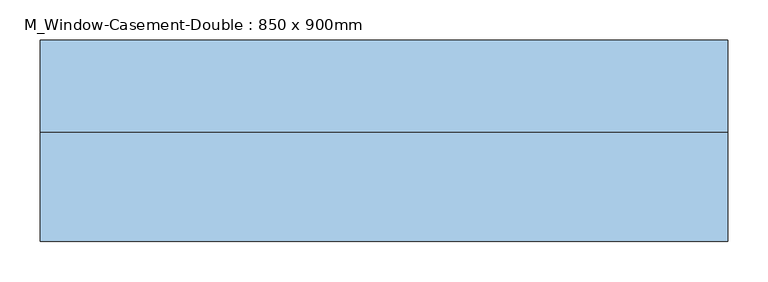
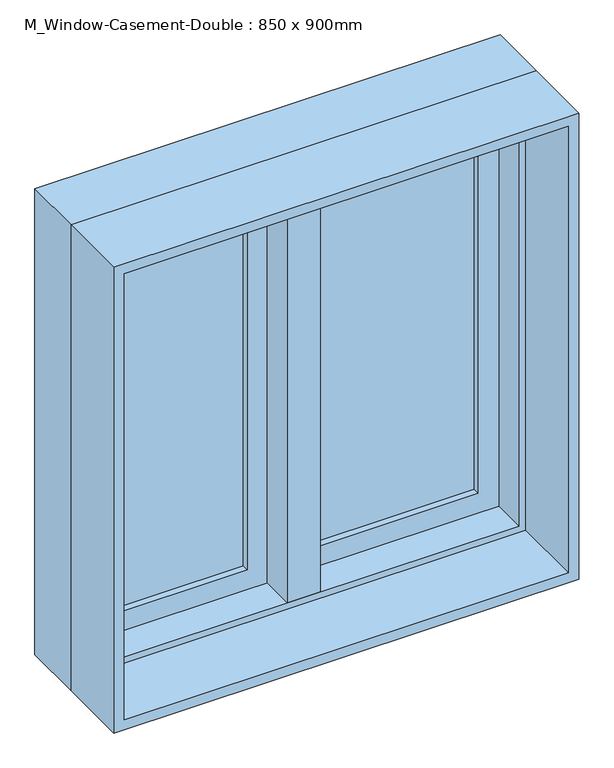
"""IFC4 building model written with IfcOpenShell, lengths in millimetres: window geometry, M_Window-Casement-Double : 850 x 900mm."""

from ifc_helpers import new_model, si_unit, frame, origin, place, context, project, spatial, polyline, outline, extrude, faceted_brep, source, transform, mapped, element, save


def m_window_casement_double_850_x_900mm_c1c4159e(model_context):
    return source(origin(), model_context, "Body", "SolidModel", [
        faceted_brep([(9.525, 134.05, 1787.3), (-9.525, 134.05, 1787.3), (-9.525, 83.25, 1787.3), (9.525, 83.25, 1787.3), (9.525, 134.05, 912.7), (9.525, 83.25, 912.7), (-9.525, 83.25, 912.7), (-9.525, 134.05, 912.7), (-9.525, 83.25, 931.75), (-9.525, 83.25, 1768.25), (-30.1625, 83.25, 931.75), (-30.1625, 83.25, 1768.25), (-30.1625, 19.75, 931.75), (-30.1625, 19.75, 1768.25), (30.1625, 19.75, 931.75), (30.1625, 19.75, 1768.25), (30.1625, 83.25, 931.75), (30.1625, 83.25, 1768.25), (9.525, 83.25, 931.75), (9.525, 83.25, 1768.25)], [[[0, 1, 2, 3]], [[4, 5, 6, 7]], [[1, 0, 4, 7]], [[2, 1, 7, 6, 8, 9]], [[9, 8, 10, 11]], [[11, 10, 12, 13]], [[13, 12, 14, 15]], [[15, 14, 16, 17]], [[17, 16, 18, 19]], [[0, 3, 19, 18, 5, 4]], [[18, 8, 6, 5]], [[9, 19, 3, 2]], [[8, 18, 16, 14, 12, 10]], [[19, 9, 11, 13, 15, 17]]]),
        extrude(outline(polyline([(-66.675, 115.0), (-66.675, 108.65), (-355.15, 108.65), (-355.15, 115.0), (-66.675, 115.0)])), frame((0.0, 0.0, 969.85), z_axis=(0.0, 0.0, 1.0), x_axis=(1.0, 0.0, 0.0)), (0.0, 0.0, 1.0), 760.3),
        extrude(outline(polyline([(-355.15, 95.95), (-355.15, 102.3), (-66.675, 102.3), (-66.675, 95.95), (-355.15, 95.95)])), frame((0.0, 0.0, 969.85), z_axis=(0.0, 0.0, 1.0), x_axis=(1.0, 0.0, 0.0)), (0.0, 0.0, 1.0), 760.3),
        extrude(outline(polyline([(355.15, 115.0), (355.15, 108.65), (66.675, 108.65), (66.675, 115.0), (355.15, 115.0)])), frame((0.0, 0.0, 969.85), z_axis=(0.0, 0.0, 1.0), x_axis=(1.0, 0.0, 0.0)), (0.0, 0.0, 1.0), 760.3),
        extrude(outline(polyline([(66.675, 95.95), (66.675, 102.3), (355.15, 102.3), (355.15, 95.95), (66.675, 95.95)])), frame((0.0, 0.0, 969.85), z_axis=(0.0, 0.0, 1.0), x_axis=(1.0, 0.0, 0.0)), (0.0, 0.0, 1.0), 760.3),
        extrude(outline(polyline([(1787.3, -412.3), (912.7, -412.3), (912.7, -9.525), (1787.3, -9.525), (1787.3, -412.3)]), holes=[polyline([(1730.15, -66.675), (969.85, -66.675), (969.85, -355.15), (1730.15, -355.15), (1730.15, -66.675)])]), frame((0.0, 83.25, 0.0), z_axis=(0.0, 1.0, 0.0), x_axis=(0.0, 0.0, 1.0)), (0.0, 0.0, 1.0), 44.45),
        extrude(outline(polyline([(912.7, 412.3), (1787.3, 412.3), (1787.3, 9.525), (912.7, 9.525), (912.7, 412.3)]), holes=[polyline([(969.85, 66.675), (1730.15, 66.675), (1730.15, 355.15), (969.85, 355.15), (969.85, 66.675)])]), frame((0.0, 83.25, 0.0), z_axis=(0.0, 1.0, 0.0), x_axis=(0.0, 0.0, 1.0)), (0.0, 0.0, 1.0), 44.45),
        extrude(outline(polyline([(1800.0, -425.0), (900.0, -425.0), (900.0, 425.0), (1800.0, 425.0), (1800.0, -425.0)]), holes=[polyline([(1780.95, 405.95), (919.05, 405.95), (919.05, -405.95), (1780.95, -405.95), (1780.95, 405.95)])]), frame((0.0, -115.0, 0.0), z_axis=(0.0, 1.0, 0.0), x_axis=(0.0, 0.0, 1.0)), (0.0, 0.0, 1.0), 134.75),
        faceted_brep([(393.25, 83.25, 1768.25), (393.25, 19.75, 1768.25), (-393.25, 19.75, 1768.25), (-393.25, 83.25, 1768.25), (412.3, 134.05, 1787.3), (412.3, 83.25, 1787.3), (-412.3, 83.25, 1787.3), (-412.3, 134.05, 1787.3), (425.0, 19.75, 1800.0), (425.0, 134.05, 1800.0), (-425.0, 134.05, 1800.0), (-425.0, 19.75, 1800.0), (-393.25, 19.75, 931.75), (-393.25, 83.25, 931.75), (-412.3, 83.25, 912.7), (-412.3, 134.05, 912.7), (-425.0, 134.05, 900.0), (-425.0, 19.75, 900.0), (393.25, 19.75, 931.75), (393.25, 83.25, 931.75), (412.3, 83.25, 912.7), (412.3, 134.05, 912.7), (425.0, 134.05, 900.0), (425.0, 19.75, 900.0)], [[[0, 1, 2, 3]], [[4, 5, 6, 7]], [[8, 9, 10, 11]], [[3, 2, 12, 13]], [[7, 6, 14, 15]], [[11, 10, 16, 17]], [[13, 12, 18, 19]], [[15, 14, 20, 21]], [[17, 16, 22, 23]], [[11, 17, 23, 8], [1, 18, 12, 2]], [[19, 18, 1, 0]], [[5, 20, 14, 6], [3, 13, 19, 0]], [[21, 20, 5, 4]], [[23, 22, 9, 8]], [[9, 22, 16, 10], [7, 15, 21, 4]]]),
    ])


if __name__ == "__main__":
    model = new_model("IFC4")
    model_context = context("Model", 3, world=origin())
    ifc_project = project(units=[si_unit("LENGTHUNIT", "METRE", prefix="MILLI")], contexts=[model_context])
    site = spatial("IfcSite", under=ifc_project)
    building = spatial("IfcBuilding", under=site)
    placement = place(None, origin())
    m_window_casement_double_850_x_900mm_shape = m_window_casement_double_850_x_900mm_c1c4159e(model_context)
    element("IfcWindow", 1, ObjectType="M_Window-Casement-Double : 850 x 900mm", at=placement, inside=building, context=model_context, shape_type="MappedRepresentation", body=[
        mapped(m_window_casement_double_850_x_900mm_shape, transform((0.0, 0.0, 0.0), x_axis=(1.0, 0.0, 0.0), y_axis=(0.0, 1.0, 0.0), z_axis=(0.0, 0.0, 1.0))),
    ])
    save(model, "model.ifc")

# Revit data of these elements
# Type "M_Window-Casement-Double : 850 x 900mm"
#   Type Mark = "23"
#   Fire Rating = "0.5h"
#   Assembly Code = "B2020100"
#   Analytic Construction = "Double glazing - domestic"
#   Frame Extension [instance default] = 0.635 cm
#   Window Inset [instance default] = 0 cm
#   Wall Thickness [instance default] = 15 cm
#   Interior Wall Closure [instance default] = 5.475 cm
#   Half Width = 42.5 cm
#   Visual Light Transmittance = 0.81
#   Thermal Resistance (R) = 0.319569 (m²·K)/W
#   Solar Heat Gain Coefficient = 0.76
#   Rough Width = 86.5 cm
#   Rough Height = 91.5 cm
#   Height = 90 cm
#   Heat Transfer Coefficient (U) = 3.12929 W/(m²·K)
#   Exterior Wall Closure [instance default] = 3.18 cm
#   Extension Jamb [instance default] = 5.475 cm
#   Default Sill Height = 90 cm
#   Width = 85 cm
#   Muntin Visibility = yes
#   Interior Trim Visibility [instance default] = yes
#   Exterior Trim Visibility [instance default] = yes
#   Extension Jamb Visibility [instance default] = yes
#   Interior Trim Material = Wood - Stained
#   Muntin Pattern = M_Muntin Pattern_2x2 : M_Muntin Pattern_2x2
#   Interior Trim = M_Trim-Window-Interior-Flat : Picture Frame
#   Interior Frame Material = Wood - Stained
#   Glass Panel Material = Glass
#   Exterior Trim Material = Clad - White
#   Exterior Trim = M_Trim-Window-Exterior-Flat : with Sill
#   Exterior Frame Material = Clad - White
#   Wall Closure = (empty or 0)
# Element 1 (IfcWindow, "M_Window-Casement-Double : 850 x 900mm")
#   Wall Thickness = 23 cm
#   Extension Jamb = 13.475 cm
#   Materials on its faces: "Wood - Stained", "Glass", "Clad - White"
# Materials
#   "Wood - Stained": class "Wood", colour RGB 224 178 126, transparency 0, Cost = 0
#   "Glass": class "Glass", colour RGB 0 128 192, transparency 0.9, Description = "Soda Lime Glass", Cost = 0
#   "Clad - White": class "Wood", colour RGB 242 242 238, transparency 0, Cost = 0
